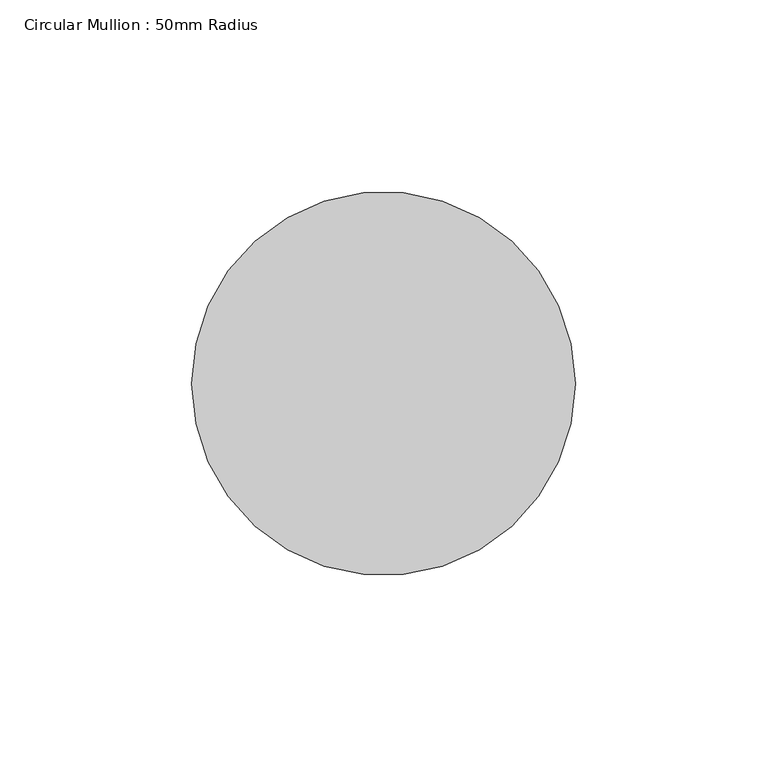
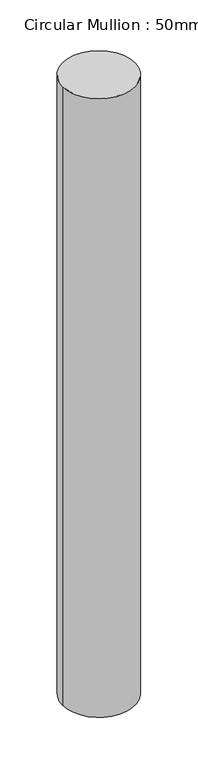
"""IFC4 building model written with IfcOpenShell, lengths in millimetres: member geometry, Circular Mullion : 50mm Radius."""

from ifc_helpers import new_model, si_unit, point, frame, origin, origin_2d, place, context, project, spatial, circle_curve, trimmed, segment, composite_curve, outline, extrude, source, transform, mapped, element, save


def circular_mullion_50mm_radius_8b077b98(model_context):
    return source(origin(), model_context, "Body", "SweptSolid", [
        extrude(outline(composite_curve([segment(trimmed(circle_curve(origin_2d(), 50.0), [point((50.0, 0.0))], [point((-50.0, 0.0))], False, "CARTESIAN"), True, "CONTINUOUS"), segment(trimmed(circle_curve(origin_2d(), 50.0), [point((-50.0, 0.0))], [point((50.0, 0.0))], False, "CARTESIAN"), True, "CONTINUOUS")], self_intersect=False)), frame((0.0, 0.0, -902.3413006), z_axis=(0.0, 0.0, 1.0), x_axis=(1.0, 0.0, 0.0)), (0.0, 0.0, 1.0), 902.3413006),
    ])


if __name__ == "__main__":
    model = new_model("IFC4")
    model_context = context("Model", 3, world=origin())
    ifc_project = project(units=[si_unit("LENGTHUNIT", "METRE", prefix="MILLI")], contexts=[model_context])
    site = spatial("IfcSite", under=ifc_project)
    building = spatial("IfcBuilding", under=site)
    placement = place(None, origin())
    circular_mullion_50mm_radius_shape = circular_mullion_50mm_radius_8b077b98(model_context)
    element("IfcMember", 1, ObjectType="Circular Mullion : 50mm Radius", at=placement, inside=building, context=model_context, shape_type="MappedRepresentation", body=[
        mapped(circular_mullion_50mm_radius_shape, transform((0.0, 0.0, 0.0), x_axis=(1.0, 0.0, 0.0), y_axis=(0.0, 1.0, 0.0), z_axis=(0.0, 0.0, 1.0))),
    ])
    save(model, "model.ifc")

# Revit data of these elements
# Type "Circular Mullion : 50mm Radius"
#   built-in parameter 1007350 = 0.164042 (stored number, unit not read)
# Element 1 (IfcMember, "Circular Mullion : 50mm Radius")
#   Materials on its faces: "Aluminium"
# Materials
#   "Aluminium": class "Metal", colour RGB 247 247 247, transparency 0, Description = "Aluminium 6061", Cost = 0
